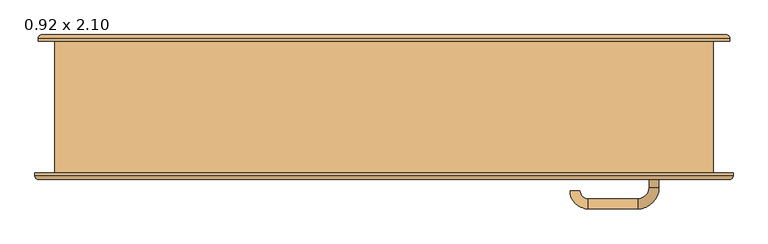
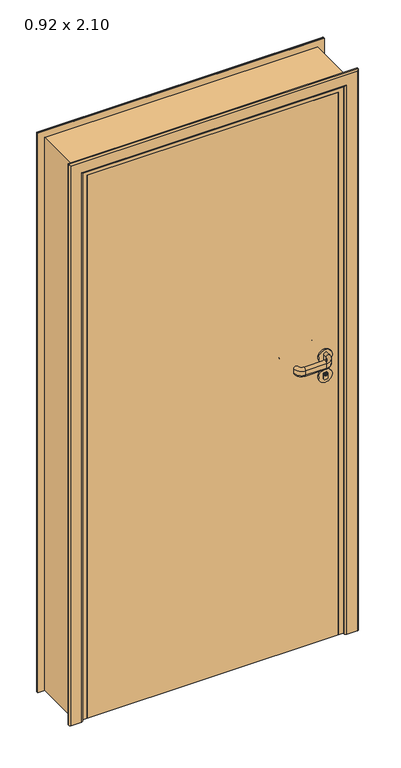
"""IFC4 building model written with IfcOpenShell, lengths in millimetres: door geometry, CC_PORTA ABRIR_1 FOLHA LISA : 0.92 x 2.10."""

from ifc_helpers import new_model, si_unit, point, frame, frame_2d, origin, origin_with_axes, place, context, project, spatial, polyline, circle_curve, ellipse_curve, trimmed, segment, composite_curve, outline, extrude, faceted_brep, source, transform, mapped, element, save
from ifc_brep_helpers import plane_surface, cylinder_surface, revolved_surface, advanced_brep


def door_0_92_x_2_10_674eabb3(model_context):
    return source(origin(), model_context, "Body", "SolidModel", [
        advanced_brep(
        [(402.5, -65.0, 1091.5062746), (417.5, -65.0, 1091.5062746), (417.5, -65.0, 1108.3826844), (402.5, -65.0, 1108.3826844), (417.5, -43.0, 1091.5062746), (417.5, -43.0, 1108.3826844), (402.5, -43.0, 1108.3826844), (402.5, -43.0, 1091.5062746), (385.0, -10.5, 1108.3826844), (385.0, -10.5, 1091.5062746), (310.0, -10.5, 1091.5062746), (310.0, -10.5, 1108.3826844), (385.0, -25.5, 1091.5062746), (385.0, -25.5, 1108.3826844), (310.0, -25.5, 1108.3826844), (310.0, -25.5, 1091.5062746), (297.5, -38.0, 1091.5062746), (297.5, -38.0, 1108.3826844), (282.5, -38.0, 1108.3826844), (282.5, -38.0, 1091.5062746)],
        [
            (0, 1, circle_curve(frame((410.0, -65.0, 1091.5062746), z_axis=(0.0, -1.0, 0.0), x_axis=(0.0, 0.0, 1.0)), 7.5)),
            (1, 2),
            (2, 3, circle_curve(frame((410.0, -65.0, 1108.3826844), z_axis=(0.0, -1.0, 0.0), x_axis=(0.0, 0.0, 1.0)), 7.5)),
            (3, 0),
            (1, 4),
            (4, 5),
            (5, 2),
            (3, 6),
            (6, 7),
            (7, 0),
            (8, 9),
            (9, 10),
            (10, 11),
            (11, 8),
            (12, 13),
            (13, 14),
            (14, 15),
            (15, 12),
            (7, 4, circle_curve(frame((410.0, -43.0, 1091.5062746), z_axis=(0.0, -1.0, 0.0), x_axis=(0.0, 0.0, 1.0)), 7.5)),
            (5, 6, circle_curve(frame((410.0, -43.0, 1108.3826844), z_axis=(0.0, -1.0, 0.0), x_axis=(0.0, 0.0, 1.0)), 7.5)),
            (9, 12, circle_curve(frame((385.0, -18.0, 1091.5062746), z_axis=(-1.0, 0.0, 0.0), x_axis=(0.0, 0.0, 1.0)), 7.5)),
            (15, 10, circle_curve(frame((310.0, -18.0, 1091.5062746), z_axis=(1.0, 0.0, 0.0), x_axis=(0.0, 0.0, 1.0)), 7.5)),
            (13, 8, circle_curve(frame((385.0, -18.0, 1108.3826844), z_axis=(-1.0, 0.0, 0.0), x_axis=(0.0, 0.0, 1.0)), 7.5)),
            (11, 14, circle_curve(frame((310.0, -18.0, 1108.3826844), z_axis=(1.0, 0.0, 0.0), x_axis=(0.0, 0.0, 1.0)), 7.5)),
            (9, 4, circle_curve(frame((385.0, -43.0, 1091.5062746), z_axis=(0.0, 0.0, -1.0), x_axis=(1.0, 0.0, 0.0)), 32.5)),
            (7, 12, circle_curve(frame((385.0, -43.0, 1091.5062746), z_axis=(0.0, 0.0, 1.0), x_axis=(1.0, 0.0, 0.0)), 17.5)),
            (8, 5, circle_curve(frame((385.0, -43.0, 1108.3826844), z_axis=(0.0, 0.0, -1.0), x_axis=(1.0, 0.0, 0.0)), 32.5)),
            (13, 6, circle_curve(frame((385.0, -43.0, 1108.3826844), z_axis=(0.0, 0.0, -1.0), x_axis=(1.0, 0.0, 0.0)), 17.5)),
            (16, 17),
            (17, 18, circle_curve(frame((290.0, -38.0, 1108.3826844), z_axis=(0.0, -1.0, 0.0), x_axis=(0.0, 0.0, 1.0)), 7.5)),
            (18, 19),
            (19, 16, circle_curve(frame((290.0, -38.0, 1091.5062746), z_axis=(0.0, -1.0, 0.0), x_axis=(0.0, 0.0, 1.0)), 7.5)),
            (19, 10, circle_curve(frame((310.0, -38.0, 1091.5062746), z_axis=(0.0, 0.0, -1.0), x_axis=(0.0, 1.0, 0.0)), 27.5)),
            (15, 16, circle_curve(frame((310.0, -38.0, 1091.5062746), z_axis=(0.0, 0.0, 1.0), x_axis=(0.0, 1.0, 0.0)), 12.5)),
            (18, 11, circle_curve(frame((310.0, -38.0, 1108.3826844), z_axis=(0.0, 0.0, -1.0), x_axis=(0.0, 1.0, 0.0)), 27.5)),
            (17, 14, circle_curve(frame((310.0, -38.0, 1108.3826844), z_axis=(0.0, 0.0, -1.0), x_axis=(0.0, 1.0, 0.0)), 12.5)),
        ],
        [
            plane_surface(frame((410.0, -65.0, 1099.9444795), z_axis=(0.0, -1.0, 0.0), x_axis=(0.0, 0.0, 1.0))),
            plane_surface(frame((417.5, -65.0, 1091.5062746), z_axis=(1.0, 0.0, 0.0), x_axis=(0.0, 1.0, 0.0))),
            plane_surface(frame((402.5, -65.0, 1108.3826844), z_axis=(-1.0, 0.0, 0.0), x_axis=(0.0, 1.0, 0.0))),
            plane_surface(frame((385.0, -10.5, 1091.5062746), z_axis=(0.0, 1.0, 0.0), x_axis=(-1.0, 0.0, 0.0))),
            plane_surface(frame((385.0, -25.5, 1108.3826844), z_axis=(0.0, -1.0, 0.0), x_axis=(-1.0, 0.0, 0.0))),
            cylinder_surface(frame((410.0, -65.0, 1091.5062746), z_axis=(0.0, -1.0, 0.0), x_axis=(0.0, 0.0, 1.0)), 7.5),
            cylinder_surface(frame((410.0, -65.0, 1108.3826844), z_axis=(0.0, -1.0, 0.0), x_axis=(0.0, 0.0, 1.0)), 7.5),
            cylinder_surface(frame((385.0, -18.0, 1091.5062746), z_axis=(1.0, 0.0, 0.0), x_axis=(0.0, 0.0, 1.0)), 7.5),
            cylinder_surface(frame((385.0, -18.0, 1108.3826844), z_axis=(1.0, 0.0, 0.0), x_axis=(0.0, 0.0, 1.0)), 7.5),
            revolved_surface(trimmed(ellipse_curve(frame((410.0, -43.0, 1091.5062746), z_axis=(0.0, -1.0, 0.0), x_axis=(0.0, 0.0, 1.0)), 7.5, 7.5), [point((402.5, -43.0, 1091.5062746))], [point((417.5, -43.0, 1091.5062746))], True, "CARTESIAN"), (385.0, -43.0, 1099.9444795), (0.0, 0.0, 1.0)),
            cylinder_surface(frame((385.0, -43.0, 1099.9444795), z_axis=(0.0, 0.0, 1.0), x_axis=(1.0, 0.0, 0.0)), 32.5),
            revolved_surface(trimmed(ellipse_curve(frame((410.0, -43.0, 1108.3826844), z_axis=(0.0, -1.0, 0.0), x_axis=(0.0, 0.0, 1.0)), 7.5, 7.5), [point((417.5, -43.0, 1108.3826844))], [point((402.5, -43.0, 1108.3826844))], True, "CARTESIAN"), (385.0, -43.0, 1099.9444795), (0.0, 0.0, 1.0)),
            revolved_surface(polyline([(402.5, -43.0, 1108.3826844), (402.5, -43.0, 1091.5062746)]), (385.0, -43.0, 1099.9444795), (0.0, 0.0, 1.0)),
            plane_surface(frame((290.0, -38.0, 1099.9444795), z_axis=(0.0, -1.0, 0.0), x_axis=(0.0, 0.0, 1.0))),
            revolved_surface(trimmed(ellipse_curve(frame((310.0, -18.0, 1091.5062746), z_axis=(1.0, 0.0, 0.0), x_axis=(0.0, 0.0, 1.0)), 7.5, 7.5), [point((310.0, -25.5, 1091.5062746))], [point((310.0, -10.5, 1091.5062746))], True, "CARTESIAN"), (310.0, -38.0, 1099.9444795), (0.0, 0.0, 1.0)),
            cylinder_surface(frame((310.0, -38.0, 1099.9444795), z_axis=(0.0, 0.0, 1.0), x_axis=(0.0, 1.0, 0.0)), 27.5),
            revolved_surface(trimmed(ellipse_curve(frame((310.0, -18.0, 1108.3826844), z_axis=(1.0, 0.0, 0.0), x_axis=(0.0, 0.0, 1.0)), 7.5, 7.5), [point((310.0, -10.5, 1108.3826844))], [point((310.0, -25.5, 1108.3826844))], True, "CARTESIAN"), (310.0, -38.0, 1099.9444795), (0.0, 0.0, 1.0)),
            revolved_surface(polyline([(310.0, -25.5, 1108.3826844), (310.0, -25.5, 1091.5062746)]), (310.0, -38.0, 1099.9444795), (0.0, 0.0, 1.0)),
        ],
        [
            (0, [[1, 2, 3, 4]]),
            (1, [[-2, 5, 6, 7]]),
            (2, [[-4, 8, 9, 10]]),
            (3, [[11, 12, 13, 14]]),
            (4, [[15, 16, 17, 18]]),
            (5, [[-1, -10, 19, -5]]),
            (6, [[-3, -7, 20, -8]]),
            (7, [[21, -18, 22, -12]]),
            (8, [[23, -14, 24, -16]]),
            (9, [[25, -19, 26, -21]]),
            (10, [[27, -6, -25, -11]]),
            (11, [[28, -20, -27, -23]]),
            (12, [[-26, -9, -28, -15]]),
            (13, [[29, 30, 31, 32]]),
            (14, [[33, -22, 34, -32]]),
            (15, [[35, -13, -33, -31]]),
            (16, [[36, -24, -35, -30]]),
            (17, [[-34, -17, -36, -29]]),
        ],
    ),
        extrude(outline(polyline([(411.0, -65.0), (409.0, -65.0), (409.0, -55.9), (411.0, -55.9), (411.0, -65.0)])), frame((0.0, 0.0, 1027.9555433), z_axis=(0.0, 0.0, 1.0), x_axis=(1.0, 0.0, 0.0)), (0.0, 0.0, 1.0), 7.8071257),
        extrude(outline(composite_curve([segment(trimmed(circle_curve(frame_2d((1031.5611613, 410.0)), 5.0), [point((1036.5611613, 410.0))], [point((1026.5611613, 410.0))], False, "CARTESIAN"), True, "CONTINUOUS"), segment(trimmed(circle_curve(frame_2d((1031.5611613, 410.0)), 5.0), [point((1026.5611613, 410.0))], [point((1036.5611613, 410.0))], False, "CARTESIAN"), True, "CONTINUOUS")], self_intersect=False), holes=[polyline([(1035.7626689, 411.0), (1027.9555433, 411.0), (1027.9555433, 409.0), (1035.7626689, 409.0), (1035.7626689, 411.0)])]), frame((0.0, -65.0, 0.0), z_axis=(0.0, 1.0, 0.0), x_axis=(0.0, 0.0, 1.0)), (0.0, 0.0, 1.0), 10.0),
        extrude(outline(composite_curve([segment(polyline([(1033.4817325, 402.5), (1016.4817325, 402.5)]), True, "CONTINUOUS"), segment(trimmed(circle_curve(frame_2d((1016.4817325, 406.5)), 4.0), [point((1016.4817325, 402.5))], [point((1012.4817325, 406.5))], False, "CARTESIAN"), True, "CONTINUOUS"), segment(polyline([(1012.4817325, 406.5), (1012.4817325, 413.5)]), True, "CONTINUOUS"), segment(trimmed(circle_curve(frame_2d((1016.4817325, 413.5)), 4.0), [point((1012.4817325, 413.5))], [point((1016.4817325, 417.5))], False, "CARTESIAN"), True, "CONTINUOUS"), segment(polyline([(1016.4817325, 417.5), (1033.4817325, 417.5)]), True, "CONTINUOUS"), segment(trimmed(circle_curve(frame_2d((1033.4817325, 413.5)), 4.0), [point((1033.4817325, 417.5))], [point((1037.4817325, 413.5))], False, "CARTESIAN"), True, "CONTINUOUS"), segment(polyline([(1037.4817325, 413.5), (1037.4817325, 406.5)]), True, "CONTINUOUS"), segment(trimmed(circle_curve(frame_2d((1033.4817325, 406.5)), 4.0), [point((1037.4817325, 406.5))], [point((1033.4817325, 402.5))], False, "CARTESIAN"), True, "CONTINUOUS")], self_intersect=False)), frame((0.0, -65.0, 0.0), z_axis=(0.0, 1.0, 0.0), x_axis=(0.0, 0.0, 1.0)), (0.0, 0.0, 1.0), 9.0),
        extrude(outline(composite_curve([segment(trimmed(circle_curve(frame_2d((1099.9444795, 410.0)), 25.0), [point((1124.9444795, 410.0))], [point((1074.9444795, 410.0))], False, "CARTESIAN"), True, "CONTINUOUS"), segment(trimmed(circle_curve(frame_2d((1099.9444795, 410.0)), 25.0), [point((1074.9444795, 410.0))], [point((1124.9444795, 410.0))], False, "CARTESIAN"), True, "CONTINUOUS")], self_intersect=False)), frame((0.0, -65.0, 0.0), z_axis=(0.0, 1.0, 0.0), x_axis=(0.0, 0.0, 1.0)), (0.0, 0.0, 1.0), 6.0),
        extrude(outline(composite_curve([segment(trimmed(circle_curve(frame_2d((1024.9444795, 410.0)), 25.0), [point((1049.9444795, 410.0))], [point((999.9444795, 410.0))], False, "CARTESIAN"), True, "CONTINUOUS"), segment(trimmed(circle_curve(frame_2d((1024.9444795, 410.0)), 25.0), [point((999.9444795, 410.0))], [point((1049.9444795, 410.0))], False, "CARTESIAN"), True, "CONTINUOUS")], self_intersect=False), holes=[composite_curve([segment(trimmed(circle_curve(frame_2d((1033.4817325, 413.5)), 4.0), [point((1037.4817325, 413.5))], [point((1033.4817325, 417.5))], True, "CARTESIAN"), True, "CONTINUOUS"), segment(polyline([(1033.4817325, 417.5), (1016.4817325, 417.5)]), True, "CONTINUOUS"), segment(trimmed(circle_curve(frame_2d((1016.4817325, 413.5)), 4.0), [point((1016.4817325, 417.5))], [point((1012.4817325, 413.5))], True, "CARTESIAN"), True, "CONTINUOUS"), segment(polyline([(1012.4817325, 413.5), (1012.4817325, 406.5)]), True, "CONTINUOUS"), segment(trimmed(circle_curve(frame_2d((1016.4817325, 406.5)), 4.0), [point((1012.4817325, 406.5))], [point((1016.4817325, 402.5))], True, "CARTESIAN"), True, "CONTINUOUS"), segment(polyline([(1016.4817325, 402.5), (1033.4817325, 402.5)]), True, "CONTINUOUS"), segment(trimmed(circle_curve(frame_2d((1033.4817325, 406.5)), 4.0), [point((1033.4817325, 402.5))], [point((1037.4817325, 406.5))], True, "CARTESIAN"), True, "CONTINUOUS"), segment(polyline([(1037.4817325, 406.5), (1037.4817325, 413.5)]), True, "CONTINUOUS")], self_intersect=False)]), frame((0.0, -65.0, 0.0), z_axis=(0.0, 1.0, 0.0), x_axis=(0.0, 0.0, 1.0)), (0.0, 0.0, 1.0), 6.0),
        extrude(outline(polyline([(411.0, -109.1), (409.0, -109.1), (409.0, -100.0), (411.0, -100.0), (411.0, -109.1)])), frame((0.0, 0.0, 1027.9555433), z_axis=(0.0, 0.0, 1.0), x_axis=(1.0, 0.0, 0.0)), (0.0, 0.0, 1.0), 7.8071257),
        advanced_brep(
        [(410.0, -110.0, 1036.5611613), (410.0, -110.0, 1026.5611613), (411.0, -110.0, 1035.7626689), (411.0, -110.0, 1027.9555433), (409.0, -110.0, 1027.9555433), (409.0, -110.0, 1035.7626689), (410.0, -100.0, 1049.9444795), (410.0, -100.0, 999.9444795), (410.0, -109.0, 1036.5611613), (410.0, -109.0, 1026.5611613), (411.0, -109.0, 1035.7626689), (411.0, -109.0, 1027.9555433), (409.0, -109.0, 1027.9555433), (409.0, -109.0, 1035.7626689), (402.5, -109.0, 1033.4817325), (402.5, -109.0, 1016.4817325), (406.5, -109.0, 1012.4817325), (413.5, -109.0, 1012.4817325), (417.5, -109.0, 1016.4817325), (417.5, -109.0, 1033.4817325), (413.5, -109.0, 1037.4817325), (406.5, -109.0, 1037.4817325), (402.5, -106.0, 1033.4817325), (402.5, -106.0, 1016.4817325), (406.5, -106.0, 1012.4817325), (413.5, -106.0, 1012.4817325), (417.5, -106.0, 1016.4817325), (417.5, -106.0, 1033.4817325), (413.5, -106.0, 1037.4817325), (406.5, -106.0, 1037.4817325), (410.0, -106.0, 1049.9444795), (410.0, -106.0, 999.9444795)],
        [
            (0, 1, circle_curve(frame((410.0, -110.0, 1031.5611613), z_axis=(0.0, -1.0, 0.0), x_axis=(0.0, 0.0, -1.0)), 5.0)),
            (1, 0, circle_curve(frame((410.0, -110.0, 1031.5611613), z_axis=(0.0, -1.0, 0.0), x_axis=(0.0, 0.0, -1.0)), 5.0)),
            (2, 3),
            (3, 4),
            (4, 5),
            (5, 2),
            (6, 7, circle_curve(frame((410.0, -100.0, 1024.9444795), z_axis=(0.0, 1.0, 0.0), x_axis=(0.0, 0.0, -1.0)), 25.0)),
            (7, 6, circle_curve(frame((410.0, -100.0, 1024.9444795), z_axis=(0.0, 1.0, 0.0), x_axis=(0.0, 0.0, -1.0)), 25.0)),
            (0, 8),
            (8, 9, circle_curve(frame((410.0, -109.0, 1031.5611613), z_axis=(0.0, -1.0, 0.0), x_axis=(0.0, 0.0, -1.0)), 5.0)),
            (9, 1),
            (9, 8, circle_curve(frame((410.0, -109.0, 1031.5611613), z_axis=(0.0, -1.0, 0.0), x_axis=(0.0, 0.0, -1.0)), 5.0)),
            (2, 10),
            (10, 11),
            (11, 3),
            (11, 12),
            (12, 4),
            (12, 13),
            (13, 5),
            (13, 10),
            (14, 15),
            (15, 16, circle_curve(frame((406.5, -109.0, 1016.4817325), z_axis=(0.0, -1.0, 0.0), x_axis=(0.0, 0.0, -1.0)), 4.0)),
            (16, 17),
            (17, 18, circle_curve(frame((413.5, -109.0, 1016.4817325), z_axis=(0.0, -1.0, 0.0), x_axis=(0.0, 0.0, -1.0)), 4.0)),
            (18, 19),
            (19, 20, circle_curve(frame((413.5, -109.0, 1033.4817325), z_axis=(0.0, -1.0, 0.0), x_axis=(0.0, 0.0, -1.0)), 4.0)),
            (20, 21),
            (21, 14, circle_curve(frame((406.5, -109.0, 1033.4817325), z_axis=(0.0, -1.0, 0.0), x_axis=(0.0, 0.0, -1.0)), 4.0)),
            (14, 22),
            (22, 23),
            (23, 15),
            (23, 24, circle_curve(frame((406.5, -106.0, 1016.4817325), z_axis=(0.0, -1.0, 0.0), x_axis=(0.0, 0.0, -1.0)), 4.0)),
            (24, 16),
            (24, 25),
            (25, 17),
            (25, 26, circle_curve(frame((413.5, -106.0, 1016.4817325), z_axis=(0.0, -1.0, 0.0), x_axis=(0.0, 0.0, -1.0)), 4.0)),
            (26, 18),
            (26, 27),
            (27, 19),
            (27, 28, circle_curve(frame((413.5, -106.0, 1033.4817325), z_axis=(0.0, -1.0, 0.0), x_axis=(0.0, 0.0, -1.0)), 4.0)),
            (28, 20),
            (28, 29),
            (29, 21),
            (29, 22, circle_curve(frame((406.5, -106.0, 1033.4817325), z_axis=(0.0, -1.0, 0.0), x_axis=(0.0, 0.0, -1.0)), 4.0)),
            (30, 31, circle_curve(frame((410.0, -106.0, 1024.9444795), z_axis=(0.0, -1.0, 0.0), x_axis=(0.0, 0.0, -1.0)), 25.0)),
            (31, 30, circle_curve(frame((410.0, -106.0, 1024.9444795), z_axis=(0.0, -1.0, 0.0), x_axis=(0.0, 0.0, -1.0)), 25.0)),
            (30, 6),
            (7, 31),
        ],
        [
            plane_surface(frame((410.0, -110.0, 1026.5611613), z_axis=(0.0, -1.0, 0.0), x_axis=(1.0, 0.0, 0.0))),
            plane_surface(frame((410.0, -100.0, 1026.5611613), z_axis=(0.0, 1.0, 0.0), x_axis=(-1.0, 0.0, 0.0))),
            cylinder_surface(frame((410.0, -100.0, 1031.5611613), z_axis=(0.0, -1.0, 0.0), x_axis=(0.0, 0.0, -1.0)), 5.0),
            plane_surface(frame((411.0, -110.0, 1035.7626689), z_axis=(-1.0, 0.0, 0.0), x_axis=(0.0, 1.0, 0.0))),
            plane_surface(frame((411.0, -110.0, 1027.9555433), z_axis=(0.0, 0.0, 1.0), x_axis=(0.0, 1.0, 0.0))),
            plane_surface(frame((409.0, -110.0, 1027.9555433), z_axis=(1.0, 0.0, 0.0), x_axis=(0.0, 1.0, 0.0))),
            plane_surface(frame((409.0, -110.0, 1035.7626689), z_axis=(0.0, 0.0, -1.0), x_axis=(0.0, 1.0, 0.0))),
            plane_surface(frame((402.5, -109.0, 1016.4817325), z_axis=(0.0, -1.0, 0.0), x_axis=(0.0, 0.0, -1.0))),
            plane_surface(frame((402.5, -109.0, 1033.4817325), z_axis=(-1.0, 0.0, 0.0), x_axis=(0.0, 1.0, 0.0))),
            cylinder_surface(frame((406.5, -100.0, 1016.4817325), z_axis=(0.0, -1.0, 0.0), x_axis=(0.0, 0.0, -1.0)), 4.0),
            plane_surface(frame((406.5, -109.0, 1012.4817325), z_axis=(0.0, 0.0, -1.0), x_axis=(0.0, 1.0, 0.0))),
            cylinder_surface(frame((413.5, -100.0, 1016.4817325), z_axis=(0.0, -1.0, 0.0), x_axis=(0.0, 0.0, -1.0)), 4.0),
            plane_surface(frame((417.5, -109.0, 1016.4817325), z_axis=(1.0, 0.0, 0.0), x_axis=(0.0, 1.0, 0.0))),
            cylinder_surface(frame((413.5, -100.0, 1033.4817325), z_axis=(0.0, -1.0, 0.0), x_axis=(0.0, 0.0, -1.0)), 4.0),
            plane_surface(frame((413.5, -109.0, 1037.4817325), z_axis=(0.0, 0.0, 1.0), x_axis=(0.0, 1.0, 0.0))),
            cylinder_surface(frame((406.5, -100.0, 1033.4817325), z_axis=(0.0, -1.0, 0.0), x_axis=(0.0, 0.0, -1.0)), 4.0),
            plane_surface(frame((410.0, -106.0, 1074.9444795), z_axis=(0.0, -1.0, 0.0), x_axis=(1.0, 0.0, 0.0))),
            cylinder_surface(frame((410.0, -100.0, 1024.9444795), z_axis=(0.0, -1.0, 0.0), x_axis=(0.0, 0.0, -1.0)), 25.0),
        ],
        [
            (0, [[1, 2], [3, 4, 5, 6]]),
            (1, [[7, 8]]),
            (2, [[-1, 9, 10, 11]]),
            (2, [[-2, -11, 12, -9]]),
            (3, [[-3, 13, 14, 15]]),
            (4, [[-4, -15, 16, 17]]),
            (5, [[-5, -17, 18, 19]]),
            (6, [[-6, -19, 20, -13]]),
            (7, [[-14, -20, -18, -16]]),
            (7, [[21, 22, 23, 24, 25, 26, 27, 28], [-10, -12]]),
            (8, [[-21, 29, 30, 31]]),
            (9, [[-22, -31, 32, 33]]),
            (10, [[-23, -33, 34, 35]]),
            (11, [[-24, -35, 36, 37]]),
            (12, [[-25, -37, 38, 39]]),
            (13, [[-26, -39, 40, 41]]),
            (14, [[-27, -41, 42, 43]]),
            (15, [[-28, -43, 44, -29]]),
            (16, [[45, 46], [-30, -44, -42, -40, -38, -36, -34, -32]]),
            (17, [[-45, 47, -8, 48]]),
            (17, [[-46, -48, -7, -47]]),
        ],
    ),
        advanced_brep(
        [(410.0, -100.0, 1124.9444795), (410.0, -100.0, 1074.9444795), (410.0, -106.0, 1124.9444795), (410.0, -106.0, 1074.9444795)],
        [
            (0, 1, circle_curve(frame((410.0, -100.0, 1099.9444795), z_axis=(0.0, 1.0, 0.0), x_axis=(0.0, 0.0, -1.0)), 25.0)),
            (1, 0, circle_curve(frame((410.0, -100.0, 1099.9444795), z_axis=(0.0, 1.0, 0.0), x_axis=(0.0, 0.0, -1.0)), 25.0)),
            (2, 3, circle_curve(frame((410.0, -106.0, 1099.9444795), z_axis=(0.0, -1.0, 0.0), x_axis=(0.0, 0.0, -1.0)), 25.0)),
            (3, 2, circle_curve(frame((410.0, -106.0, 1099.9444795), z_axis=(0.0, -1.0, 0.0), x_axis=(0.0, 0.0, -1.0)), 25.0)),
            (2, 0),
            (1, 3),
        ],
        [
            plane_surface(frame((410.0, -100.0, 1026.5611613), z_axis=(0.0, 1.0, 0.0), x_axis=(-1.0, 0.0, 0.0))),
            plane_surface(frame((410.0, -106.0, 1074.9444795), z_axis=(0.0, -1.0, 0.0), x_axis=(1.0, 0.0, 0.0))),
            cylinder_surface(frame((410.0, -100.0, 1099.9444795), z_axis=(0.0, -1.0, 0.0), x_axis=(0.0, 0.0, -1.0)), 25.0),
        ],
        [
            (0, [[1, 2]]),
            (1, [[3, 4]]),
            (2, [[-3, 5, -2, 6]]),
            (2, [[-4, -6, -1, -5]]),
        ],
    ),
        advanced_brep(
        [(402.5, -100.0, 1108.4382049), (417.5, -100.0, 1108.4382049), (417.5, -100.0, 1091.5617951), (402.5, -100.0, 1091.5617951), (417.5, -122.0, 1108.4382049), (417.5, -122.0, 1091.5617951), (402.5, -122.0, 1091.5617951), (402.5, -122.0, 1108.4382049), (385.0, -154.5, 1091.5617951), (385.0, -154.5, 1108.4382049), (310.0, -154.5, 1108.4382049), (310.0, -154.5, 1091.5617951), (385.0, -139.5, 1108.4382049), (385.0, -139.5, 1091.5617951), (310.0, -139.5, 1091.5617951), (310.0, -139.5, 1108.4382049), (297.5, -127.0, 1108.4382049), (297.5, -127.0, 1091.5617951), (282.5, -127.0, 1091.5617951), (282.5, -127.0, 1108.4382049)],
        [
            (0, 1, circle_curve(frame((410.0, -100.0, 1108.4382049), z_axis=(0.0, 1.0, 0.0), x_axis=(-1.0, 0.0, 0.0)), 7.5)),
            (1, 2),
            (2, 3, circle_curve(frame((410.0, -100.0, 1091.5617951), z_axis=(0.0, 1.0, 0.0), x_axis=(-1.0, 0.0, 0.0)), 7.5)),
            (3, 0),
            (1, 4),
            (4, 5),
            (5, 2),
            (3, 6),
            (6, 7),
            (7, 0),
            (8, 9),
            (9, 10),
            (10, 11),
            (11, 8),
            (12, 13),
            (13, 14),
            (14, 15),
            (15, 12),
            (7, 4, circle_curve(frame((410.0, -122.0, 1108.4382049), z_axis=(0.0, 1.0, 0.0), x_axis=(-1.0, 0.0, 0.0)), 7.5)),
            (5, 6, circle_curve(frame((410.0, -122.0, 1091.5617951), z_axis=(0.0, 1.0, 0.0), x_axis=(-1.0, 0.0, 0.0)), 7.5)),
            (9, 12, circle_curve(frame((385.0, -147.0, 1108.4382049), z_axis=(-1.0, 0.0, 0.0), x_axis=(0.0, 1.0, 0.0)), 7.5)),
            (15, 10, circle_curve(frame((310.0, -147.0, 1108.4382049), z_axis=(1.0, 0.0, 0.0), x_axis=(0.0, 1.0, 0.0)), 7.5)),
            (13, 8, circle_curve(frame((385.0, -147.0, 1091.5617951), z_axis=(-1.0, 0.0, 0.0), x_axis=(0.0, 1.0, 0.0)), 7.5)),
            (11, 14, circle_curve(frame((310.0, -147.0, 1091.5617951), z_axis=(1.0, 0.0, 0.0), x_axis=(0.0, 1.0, 0.0)), 7.5)),
            (9, 4, circle_curve(frame((385.0, -122.0, 1108.4382049), z_axis=(0.0, 0.0, 1.0), x_axis=(1.0, 0.0, 0.0)), 32.5)),
            (7, 12, circle_curve(frame((385.0, -122.0, 1108.4382049), z_axis=(0.0, 0.0, -1.0), x_axis=(1.0, 0.0, 0.0)), 17.5)),
            (8, 5, circle_curve(frame((385.0, -122.0, 1091.5617951), z_axis=(0.0, 0.0, 1.0), x_axis=(1.0, 0.0, 0.0)), 32.5)),
            (13, 6, circle_curve(frame((385.0, -122.0, 1091.5617951), z_axis=(0.0, 0.0, 1.0), x_axis=(1.0, 0.0, 0.0)), 17.5)),
            (16, 17),
            (17, 18, circle_curve(frame((290.0, -127.0, 1091.5617951), z_axis=(0.0, 1.0, 0.0), x_axis=(1.0, 0.0, 0.0)), 7.5)),
            (18, 19),
            (19, 16, circle_curve(frame((290.0, -127.0, 1108.4382049), z_axis=(0.0, 1.0, 0.0), x_axis=(1.0, 0.0, 0.0)), 7.5)),
            (19, 10, circle_curve(frame((310.0, -127.0, 1108.4382049), z_axis=(0.0, 0.0, 1.0), x_axis=(0.0, -1.0, 0.0)), 27.5)),
            (15, 16, circle_curve(frame((310.0, -127.0, 1108.4382049), z_axis=(0.0, 0.0, -1.0), x_axis=(0.0, -1.0, 0.0)), 12.5)),
            (18, 11, circle_curve(frame((310.0, -127.0, 1091.5617951), z_axis=(0.0, 0.0, 1.0), x_axis=(0.0, -1.0, 0.0)), 27.5)),
            (17, 14, circle_curve(frame((310.0, -127.0, 1091.5617951), z_axis=(0.0, 0.0, 1.0), x_axis=(0.0, -1.0, 0.0)), 12.5)),
        ],
        [
            plane_surface(frame((410.0, -100.0, 1100.0), z_axis=(0.0, 1.0, 0.0), x_axis=(0.0, 0.0, -1.0))),
            plane_surface(frame((417.5, -100.0, 1108.4382049), z_axis=(1.0, 0.0, 0.0), x_axis=(0.0, -1.0, 0.0))),
            plane_surface(frame((402.5, -100.0, 1091.5617951), z_axis=(-1.0, 0.0, 0.0), x_axis=(0.0, -1.0, 0.0))),
            plane_surface(frame((385.0, -154.5, 1108.4382049), z_axis=(0.0, -1.0, 0.0), x_axis=(-1.0, 0.0, 0.0))),
            plane_surface(frame((385.0, -139.5, 1091.5617951), z_axis=(0.0, 1.0, 0.0), x_axis=(-1.0, 0.0, 0.0))),
            cylinder_surface(frame((410.0, -100.0, 1108.4382049), z_axis=(0.0, 1.0, 0.0), x_axis=(-1.0, 0.0, 0.0)), 7.5),
            cylinder_surface(frame((410.0, -100.0, 1091.5617951), z_axis=(0.0, 1.0, 0.0), x_axis=(-1.0, 0.0, 0.0)), 7.5),
            cylinder_surface(frame((385.0, -147.0, 1108.4382049), z_axis=(1.0, 0.0, 0.0), x_axis=(0.0, 1.0, 0.0)), 7.5),
            cylinder_surface(frame((385.0, -147.0, 1091.5617951), z_axis=(1.0, 0.0, 0.0), x_axis=(0.0, 1.0, 0.0)), 7.5),
            revolved_surface(trimmed(ellipse_curve(frame((410.0, -122.0, 1108.4382049), z_axis=(0.0, 1.0, 0.0), x_axis=(-1.0, 0.0, 0.0)), 7.5, 7.5), [point((402.5, -122.0, 1108.4382049))], [point((417.5, -122.0, 1108.4382049))], True, "CARTESIAN"), (385.0, -122.0, 1100.0), (0.0, 0.0, -1.0)),
            cylinder_surface(frame((385.0, -122.0, 1100.0), z_axis=(0.0, 0.0, -1.0), x_axis=(1.0, 0.0, 0.0)), 32.5),
            revolved_surface(trimmed(ellipse_curve(frame((410.0, -122.0, 1091.5617951), z_axis=(0.0, 1.0, 0.0), x_axis=(-1.0, 0.0, 0.0)), 7.5, 7.5), [point((417.5, -122.0, 1091.5617951))], [point((402.5, -122.0, 1091.5617951))], True, "CARTESIAN"), (385.0, -122.0, 1100.0), (0.0, 0.0, -1.0)),
            revolved_surface(polyline([(402.5, -122.0, 1091.5617951), (402.5, -122.0, 1108.4382049)]), (385.0, -122.0, 1100.0), (0.0, 0.0, -1.0)),
            plane_surface(frame((290.0, -127.0, 1100.0), z_axis=(0.0, 1.0, 0.0), x_axis=(0.0, 0.0, -1.0))),
            revolved_surface(trimmed(ellipse_curve(frame((310.0, -147.0, 1108.4382049), z_axis=(1.0, 0.0, 0.0), x_axis=(0.0, 1.0, 0.0)), 7.5, 7.5), [point((310.0, -139.5, 1108.4382049))], [point((310.0, -154.5, 1108.4382049))], True, "CARTESIAN"), (310.0, -127.0, 1100.0), (0.0, 0.0, -1.0)),
            cylinder_surface(frame((310.0, -127.0, 1100.0), z_axis=(0.0, 0.0, -1.0), x_axis=(0.0, -1.0, 0.0)), 27.5),
            revolved_surface(trimmed(ellipse_curve(frame((310.0, -147.0, 1091.5617951), z_axis=(1.0, 0.0, 0.0), x_axis=(0.0, 1.0, 0.0)), 7.5, 7.5), [point((310.0, -154.5, 1091.5617951))], [point((310.0, -139.5, 1091.5617951))], True, "CARTESIAN"), (310.0, -127.0, 1100.0), (0.0, 0.0, -1.0)),
            revolved_surface(polyline([(310.0, -139.5, 1091.5617951), (310.0, -139.5, 1108.4382049)]), (310.0, -127.0, 1100.0), (0.0, 0.0, -1.0)),
        ],
        [
            (0, [[1, 2, 3, 4]]),
            (1, [[-2, 5, 6, 7]]),
            (2, [[-4, 8, 9, 10]]),
            (3, [[11, 12, 13, 14]]),
            (4, [[15, 16, 17, 18]]),
            (5, [[-1, -10, 19, -5]]),
            (6, [[-3, -7, 20, -8]]),
            (7, [[21, -18, 22, -12]]),
            (8, [[23, -14, 24, -16]]),
            (9, [[25, -19, 26, -21]]),
            (10, [[27, -6, -25, -11]]),
            (11, [[28, -20, -27, -23]]),
            (12, [[-26, -9, -28, -15]]),
            (13, [[29, 30, 31, 32]]),
            (14, [[33, -22, 34, -32]]),
            (15, [[35, -13, -33, -31]]),
            (16, [[36, -24, -35, -30]]),
            (17, [[-34, -17, -36, -29]]),
        ],
    ),
        extrude(outline(polyline([(460.0, -100.0), (-460.0, -100.0), (-460.0, -65.0), (460.0, -65.0), (460.0, -100.0)])), origin_with_axes(), (0.0, 0.0, 1.0), 2100.0),
        advanced_brep(
        [(-480.5, 110.0, 0.0), (-475.0, 104.5, 0.0), (-475.0, 100.0, 0.0), (-525.0, 100.0, 0.0), (-525.0, 104.500573, 0.0), (-519.500573, 110.0, 0.0), (-480.5, 110.0, 2120.5), (-475.0, 104.5, 2115.0), (-475.0, 100.0, 2115.0), (475.0, 100.0, 2115.0), (475.0, 100.0, 0.0), (525.0, 100.0, 0.0), (525.0, 100.0, 2165.0), (-525.0, 100.0, 2165.0), (-525.0, 104.500573, 2165.0), (-519.500573, 110.0, 2159.500573), (519.500573, 110.0, 2159.500573), (519.500573, 110.0, 0.0), (480.5, 110.0, 0.0), (480.5, 110.0, 2120.5), (475.0, 104.5, 2115.0), (475.0, 104.5, 0.0), (525.0, 104.500573, 0.0), (525.0, 104.500573, 2165.0)],
        [
            (0, 1, circle_curve(frame((-480.5, 104.5, 0.0), z_axis=(0.0, 0.0, -1.0), x_axis=(0.0, 1.0, 0.0)), 5.5)),
            (1, 2),
            (2, 3),
            (3, 4),
            (4, 5, circle_curve(frame((-519.500573, 104.500573, 0.0), z_axis=(0.0, 0.0, -1.0), x_axis=(0.0, 1.0, 0.0)), 5.499427)),
            (5, 0),
            (0, 6),
            (6, 7, ellipse_curve(frame((-480.5, 104.5, 2120.5), z_axis=(-0.7071067811865475, 0.0, -0.7071067811865475), x_axis=(0.7071067811865474, 0.0, -0.7071067811865476)), 7.7781746, 5.5)),
            (7, 1),
            (7, 8),
            (8, 2),
            (8, 9),
            (9, 10),
            (10, 11),
            (11, 12),
            (12, 13),
            (13, 3),
            (13, 14),
            (14, 4),
            (14, 15, ellipse_curve(frame((-519.500573, 104.500573, 2159.500573), z_axis=(-0.7071067811865475, 0.0, -0.7071067811865475), x_axis=(0.7071067811865474, 0.0, -0.7071067811865476)), 7.7773642, 5.499427)),
            (15, 5),
            (15, 16),
            (16, 17),
            (17, 18),
            (18, 19),
            (19, 6),
            (9, 20),
            (20, 21),
            (21, 10),
            (17, 22, circle_curve(frame((519.500573, 104.500573, 0.0), z_axis=(0.0, 0.0, -1.0), x_axis=(0.0, 1.0, 0.0)), 5.499427)),
            (22, 11),
            (21, 18, circle_curve(frame((480.5, 104.5, 0.0), z_axis=(0.0, 0.0, -1.0), x_axis=(0.0, 1.0, 0.0)), 5.5)),
            (23, 12),
            (22, 23),
            (16, 23, ellipse_curve(frame((519.500573, 104.500573, 2159.500573), z_axis=(0.7071067811865475, 0.0, -0.7071067811865475), x_axis=(0.7071067811865474, 0.0, 0.7071067811865476)), 7.7773642, 5.499427)),
            (20, 19, ellipse_curve(frame((480.5, 104.5, 2120.5), z_axis=(0.7071067811865475, 0.0, -0.7071067811865475), x_axis=(0.7071067811865474, 0.0, 0.7071067811865476)), 7.7781746, 5.5)),
            (20, 7),
            (23, 14),
        ],
        [
            plane_surface(frame((-500.0, 100.0, 0.0), z_axis=(0.0, 0.0, -1.0), x_axis=(-1.0, 0.0, 0.0))),
            cylinder_surface(frame((-480.5, 104.5, 0.0), z_axis=(0.0, 0.0, -1.0), x_axis=(0.0, 1.0, 0.0)), 5.5),
            plane_surface(frame((-475.0, 104.5, 0.0), z_axis=(1.0, 0.0, 0.0), x_axis=(0.0, 0.0, 1.0))),
            plane_surface(frame((-475.0, 100.0, 0.0), z_axis=(0.0, -1.0, 0.0), x_axis=(0.0, 0.0, 1.0))),
            plane_surface(frame((-525.0, 100.0, 0.0), z_axis=(-1.0, 0.0, 0.0), x_axis=(0.0, 0.0, 1.0))),
            cylinder_surface(frame((-519.500573, 104.500573, 0.0), z_axis=(0.0, 0.0, -1.0), x_axis=(0.0, 1.0, 0.0)), 5.499427),
            plane_surface(frame((-519.500573, 110.0, 0.0), z_axis=(0.0, 1.0, 0.0), x_axis=(0.0, 0.0, 1.0))),
            plane_surface(frame((475.0, 104.5, 2115.0), z_axis=(-1.0, 0.0, 0.0), x_axis=(0.0, 0.0, -1.0))),
            plane_surface(frame((500.0, 100.0, 0.0), z_axis=(0.0, 0.0, -1.0), x_axis=(1.0, 0.0, 0.0))),
            plane_surface(frame((525.0, 100.0, 2165.0), z_axis=(1.0, 0.0, 0.0), x_axis=(0.0, 0.0, -1.0))),
            cylinder_surface(frame((519.500573, 104.500573, 2140.0), z_axis=(0.0, 0.0, 1.0), x_axis=(0.0, 1.0, 0.0)), 5.499427),
            cylinder_surface(frame((480.5, 104.5, 2140.0), z_axis=(0.0, 0.0, 1.0), x_axis=(0.0, 1.0, 0.0)), 5.5),
            cylinder_surface(frame((-500.0, 104.5, 2120.5), z_axis=(-1.0, 0.0, 0.0), x_axis=(0.0, 1.0, 0.0)), 5.5),
            plane_surface(frame((-475.0, 104.5, 2115.0), z_axis=(0.0, 0.0, -1.0), x_axis=(1.0, 0.0, 0.0))),
            plane_surface(frame((-525.0, 100.0, 2165.0), z_axis=(0.0, 0.0, 1.0), x_axis=(1.0, 0.0, 0.0))),
            cylinder_surface(frame((-500.0, 104.500573, 2159.500573), z_axis=(-1.0, 0.0, 0.0), x_axis=(0.0, 1.0, 0.0)), 5.499427),
        ],
        [
            (0, [[1, 2, 3, 4, 5, 6]]),
            (1, [[-1, 7, 8, 9]]),
            (2, [[-2, -9, 10, 11]]),
            (3, [[-3, -11, 12, 13, 14, 15, 16, 17]]),
            (4, [[-4, -17, 18, 19]]),
            (5, [[-5, -19, 20, 21]]),
            (6, [[-6, -21, 22, 23, 24, 25, 26, -7]]),
            (7, [[27, 28, 29, -13]]),
            (8, [[-24, 30, 31, -14, -29, 32]]),
            (9, [[33, -15, -31, 34]]),
            (10, [[35, -34, -30, -23]]),
            (11, [[36, -25, -32, -28]]),
            (12, [[-8, -26, -36, 37]]),
            (13, [[-10, -37, -27, -12]]),
            (14, [[-18, -16, -33, 38]]),
            (15, [[-20, -38, -35, -22]]),
        ],
    ),
        advanced_brep(
        [(-480.0, -100.0, 0.0), (-480.0, -104.5, 0.0), (-485.5, -110.0, 0.0), (-524.5, -110.0, 0.0), (-530.0, -104.5, 0.0), (-530.0, -100.0, 0.0), (-480.0, -100.0, 2120.0), (-480.0, -104.5, 2120.0), (-485.5, -110.0, 2125.5), (485.5, -110.0, 2125.5), (485.5, -110.0, 0.0), (524.5, -110.0, 0.0), (524.5, -110.0, 2164.5), (-524.5, -110.0, 2164.5), (-530.0, -104.5, 2170.0), (-530.0, -100.0, 2170.0), (530.0, -100.0, 2170.0), (530.0, -100.0, 0.0), (480.0, -100.0, 0.0), (480.0, -100.0, 2120.0), (480.0, -104.5, 2120.0), (480.0, -104.5, 0.0), (530.0, -104.5, 0.0), (530.0, -104.5, 2170.0)],
        [
            (0, 1),
            (1, 2, circle_curve(frame((-485.5, -104.5, 0.0), z_axis=(0.0, 0.0, -1.0), x_axis=(0.0, 1.0, 0.0)), 5.5)),
            (2, 3),
            (3, 4, circle_curve(frame((-524.5, -104.5, 0.0), z_axis=(0.0, 0.0, -1.0), x_axis=(0.0, 1.0, 0.0)), 5.5)),
            (4, 5),
            (5, 0),
            (0, 6),
            (6, 7),
            (7, 1),
            (7, 8, ellipse_curve(frame((-485.5, -104.5, 2125.5), z_axis=(-0.7071067811865475, 0.0, -0.7071067811865475), x_axis=(0.7071067811865474, 0.0, -0.7071067811865476)), 7.7781746, 5.5)),
            (8, 2),
            (8, 9),
            (9, 10),
            (10, 11),
            (11, 12),
            (12, 13),
            (13, 3),
            (13, 14, ellipse_curve(frame((-524.5, -104.5, 2164.5), z_axis=(-0.7071067811865475, 0.0, -0.7071067811865475), x_axis=(0.7071067811865474, 0.0, -0.7071067811865476)), 7.7781746, 5.5)),
            (14, 4),
            (14, 15),
            (15, 5),
            (15, 16),
            (16, 17),
            (17, 18),
            (18, 19),
            (19, 6),
            (9, 20, ellipse_curve(frame((485.5, -104.5, 2125.5), z_axis=(0.7071067811865475, 0.0, -0.7071067811865475), x_axis=(0.7071067811865474, 0.0, 0.7071067811865476)), 7.7781746, 5.5)),
            (20, 21),
            (21, 10, circle_curve(frame((485.5, -104.5, 0.0), z_axis=(0.0, 0.0, 1.0), x_axis=(0.0, 1.0, 0.0)), 5.5)),
            (17, 22),
            (22, 11, circle_curve(frame((524.5, -104.5, 0.0), z_axis=(0.0, 0.0, -1.0), x_axis=(0.0, 1.0, 0.0)), 5.5)),
            (21, 18),
            (23, 12, ellipse_curve(frame((524.5, -104.5, 2164.5), z_axis=(0.7071067811865475, 0.0, -0.7071067811865475), x_axis=(0.7071067811865474, 0.0, 0.7071067811865476)), 7.7781746, 5.5)),
            (22, 23),
            (16, 23),
            (20, 19),
            (20, 7),
            (23, 14),
        ],
        [
            plane_surface(frame((-500.0, -100.0, 0.0), z_axis=(0.0, 0.0, -1.0), x_axis=(-1.0, 0.0, 0.0))),
            plane_surface(frame((-480.0, -100.0, 0.0), z_axis=(1.0, 0.0, 0.0), x_axis=(0.0, 0.0, 1.0))),
            cylinder_surface(frame((-485.5, -104.5, 0.0), z_axis=(0.0, 0.0, -1.0), x_axis=(0.0, 1.0, 0.0)), 5.5),
            plane_surface(frame((-485.5, -110.0, 0.0), z_axis=(0.0, -1.0, 0.0), x_axis=(0.0, 0.0, 1.0))),
            cylinder_surface(frame((-524.5, -104.5, 0.0), z_axis=(0.0, 0.0, -1.0), x_axis=(0.0, 1.0, 0.0)), 5.5),
            plane_surface(frame((-530.0, -104.5, 0.0), z_axis=(-1.0, 0.0, 0.0), x_axis=(0.0, 0.0, 1.0))),
            plane_surface(frame((-530.0, -100.0, 0.0), z_axis=(0.0, 1.0, 0.0), x_axis=(0.0, 0.0, 1.0))),
            cylinder_surface(frame((485.5, -104.5, 2140.0), z_axis=(0.0, 0.0, 1.0), x_axis=(0.0, 1.0, 0.0)), 5.5),
            plane_surface(frame((500.0, -100.0, 0.0), z_axis=(0.0, 0.0, -1.0), x_axis=(1.0, 0.0, 0.0))),
            cylinder_surface(frame((524.5, -104.5, 2140.0), z_axis=(0.0, 0.0, 1.0), x_axis=(0.0, 1.0, 0.0)), 5.5),
            plane_surface(frame((530.0, -104.5, 2170.0), z_axis=(1.0, 0.0, 0.0), x_axis=(0.0, 0.0, -1.0))),
            plane_surface(frame((480.0, -100.0, 2120.0), z_axis=(-1.0, 0.0, 0.0), x_axis=(0.0, 0.0, -1.0))),
            plane_surface(frame((-480.0, -100.0, 2120.0), z_axis=(0.0, 0.0, -1.0), x_axis=(1.0, 0.0, 0.0))),
            cylinder_surface(frame((-500.0, -104.5, 2125.5), z_axis=(-1.0, 0.0, 0.0), x_axis=(0.0, 1.0, 0.0)), 5.5),
            cylinder_surface(frame((-500.0, -104.5, 2164.5), z_axis=(-1.0, 0.0, 0.0), x_axis=(0.0, 1.0, 0.0)), 5.5),
            plane_surface(frame((-530.0, -104.5, 2170.0), z_axis=(0.0, 0.0, 1.0), x_axis=(1.0, 0.0, 0.0))),
        ],
        [
            (0, [[1, 2, 3, 4, 5, 6]]),
            (1, [[-1, 7, 8, 9]]),
            (2, [[-2, -9, 10, 11]]),
            (3, [[-3, -11, 12, 13, 14, 15, 16, 17]]),
            (4, [[-4, -17, 18, 19]]),
            (5, [[-5, -19, 20, 21]]),
            (6, [[-6, -21, 22, 23, 24, 25, 26, -7]]),
            (7, [[27, 28, 29, -13]]),
            (8, [[-24, 30, 31, -14, -29, 32]]),
            (9, [[33, -15, -31, 34]]),
            (10, [[35, -34, -30, -23]]),
            (11, [[36, -25, -32, -28]]),
            (12, [[-8, -26, -36, 37]]),
            (13, [[-10, -37, -27, -12]]),
            (14, [[-18, -16, -33, 38]]),
            (15, [[-20, -38, -35, -22]]),
        ],
    ),
        faceted_brep([(-460.0, -65.0, 0.0), (-460.0, -100.0, 0.0), (-500.0, -100.0, 0.0), (-500.0, 100.0, 0.0), (-450.0, 100.0, 0.0), (-450.0, -65.0, 0.0), (-460.0, -65.0, 2100.0), (-460.0, -100.0, 2100.0), (460.0, -100.0, 2100.0), (460.0, -100.0, 0.0), (500.0, -100.0, 0.0), (500.0, -100.0, 2140.0), (-500.0, -100.0, 2140.0), (-500.0, 100.0, 2140.0), (500.0, 100.0, 2140.0), (500.0, 100.0, 0.0), (450.0, 100.0, 0.0), (450.0, 100.0, 2090.0), (-450.0, 100.0, 2090.0), (-450.0, -65.0, 2090.0), (450.0, -65.0, 2090.0), (450.0, -65.0, 0.0), (460.0, -65.0, 0.0), (460.0, -65.0, 2100.0)], [[[0, 1, 2, 3, 4, 5]], [[1, 0, 6, 7]], [[2, 1, 7, 8, 9, 10, 11, 12]], [[3, 2, 12, 13]], [[4, 3, 13, 14, 15, 16, 17, 18]], [[5, 4, 18, 19]], [[0, 5, 19, 20, 21, 22, 23, 6]], [[8, 23, 22, 9]], [[22, 21, 16, 15, 10, 9]], [[14, 11, 10, 15]], [[20, 17, 16, 21]], [[7, 6, 23, 8]], [[13, 12, 11, 14]], [[19, 18, 17, 20]]]),
    ])


if __name__ == "__main__":
    model = new_model("IFC4")
    model_context = context("Model", 3, world=origin())
    ifc_project = project(units=[si_unit("LENGTHUNIT", "METRE", prefix="MILLI")], contexts=[model_context])
    site = spatial("IfcSite", under=ifc_project)
    building = spatial("IfcBuilding", under=site)
    placement = place(None, origin())
    door_0_92_x_2_10_shape = door_0_92_x_2_10_674eabb3(model_context)
    element("IfcDoor", 1, ObjectType="CC_PORTA ABRIR_1 FOLHA LISA : 0.92 x 2.10", at=placement, inside=building, context=model_context, shape_type="MappedRepresentation", body=[
        mapped(door_0_92_x_2_10_shape, transform((0.0, 0.0, 0.0), x_axis=(1.0, 0.0, 0.0), y_axis=(0.0, 1.0, 0.0), z_axis=(0.0, 0.0, 1.0))),
    ])
    save(model, "model.ifc")

# Revit data of these elements
# Type "CC_PORTA ABRIR_1 FOLHA LISA : 0.92 x 2.10"
#   Type Mark = "P3"
#   Site = "www.construir.arq.br"
#   Empresa = "Cursos Construir"
#   Description = "PORTA ABRIR 1 FOLHA LISA"
#   Criado Por = "Roberto Netto"
#   Analytic Construction = "<Nenhum>"
#   Atualizado por = "Rudemberg Eloi"
#   Rough Width = 1.00 m
#   Interna [instance default] = 0.00 m
#   Largura Guarnição Interna [instance default] = 0.05 m
#   Largura Guarnição Externa [instance default] = 0.05 m
#   Largura Folha [instance default] = 0.92 m
#   Externa [instance default] = 0.00 m
#   Extensão Lateral Esquerda [instance default] = 0.03 m
#   Extensão Lateral Direita [instance default] = 0.03 m
#   Extensão Frontal [instance default] = 0.03 m
#   Espessura Soleira [instance default] = 0.02 m
#   Espessura Guarnição Interna [instance default] = 0.01 m
#   Espessura Guarnição Externa [instance default] = 0.01 m
#   Espessura Folha [instance default] = 0.035 m
#   Espessura Batente [instance default] = 0.05 m
#   Eixo Rotação Folha [instance default] = 0.04 m
#   Deslocamento Maçaneta [instance default] = 0.05 m
#   Deslocamento Fechadura [instance default] = 0.05 m
#   Desloc (Interno) [instance default] = 0.02 m
#   Desloc (Externo) [instance default] = 0.025 m
#   Rough Height = 2.14 m
#   Altura Maçaneta [instance default] = 1.10 m
#   Altura Folha [instance default] = 2.10 m
#   Altura Fechadura [instance default] = 1.00 m
#   Height = 2.14 m
#   Width = 1.00 m
#   ----SOLEIRA---- [instance default] = 0.00 m
#   ----MAÇANETA/FECHADURA---- [instance default] = 0.00 m
#   ----GUARNIÇÃO---- [instance default] = 0.00 m
#   ----FOLHA---- [instance default] = 0.00 m
#   ----EXTENSÃO---- [instance default] = 0.00 m
#   ----BATENTE---- [instance default] = 0.00 m
#   Soleira Sem Extensão [instance default] = yes
#   Soleira Com Extensão [instance default] = no
#   Soleira [instance default] = yes
#   Maçaneta / Puxador [instance default] = yes
#   Guarnição Interna [instance default] = yes
#   Guarnição Externa [instance default] = yes
#   Fechadura Separada [instance default] = no
#   Bit [instance default] = no
#   Porcent. Exibição Batente Interno [instance default] = 50
#   Porcent. Exibição Batente Externo [instance default] = 50
#   Material Bit/Soleira = .GRANITO BRANCO ITAÚNAS
#   Material Espelho/Fixação = .AÇO INOXIDÁVEL ESCOVADO
#   Material Maçaneta/Puxador = .AÇO INOXIDÁVEL ESCOVADO
#   Material Guarnição Interna = .MADEIRA COM PINTURA ESMALTE BRANCO ACETINADO
#   Material Guarnição Externa = .MADEIRA COM PINTURA ESMALTE BRANCO ACETINADO
#   Material Folha = .MADEIRA COM PINTURA ESMALTE BRANCO ACETINADO
#   Material Fechadura = .AÇO INOXIDÁVEL ESCOVADO
#   Material Batente = .MADEIRA COM PINTURA ESMALTE BRANCO ACETINADO
#   Família Maçaneta [instance default] = element 613477
#   Function = (empty or 0)
#   Wall Closure = (empty or 0)
# Element 1 (IfcDoor, "CC_PORTA ABRIR_1 FOLHA LISA : 0.92 x 2.10")
#   Materials on its faces: ".AÇO INOXIDÁVEL ESCOVADO", ".MADEIRA COM PINTURA ESMALTE BRANCO ACETINADO"
# Materials
#   ".GRANITO BRANCO ITAÚNAS": class ".CC_PEDRA REVEST.", colour RGB 202 195 174, transparency 0, Description = "Granito branco Itaúnas", Uso = "Pedra", Cost = 0
#   ".AÇO INOXIDÁVEL ESCOVADO": class "Metal", colour RGB 189 187 185, transparency 0, Description = "Stainless Steel 18/8, brushed finish", Cost = 0
#   ".MADEIRA COM PINTURA ESMALTE BRANCO ACETINADO": class ".CC_MADEIRAS", colour RGB 240 240 240, transparency 0, Description = "Madeira com pintura esmalte branco acetinado.", Cost = 0
